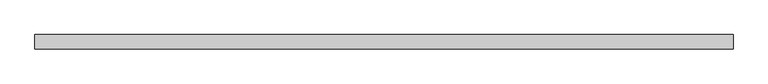
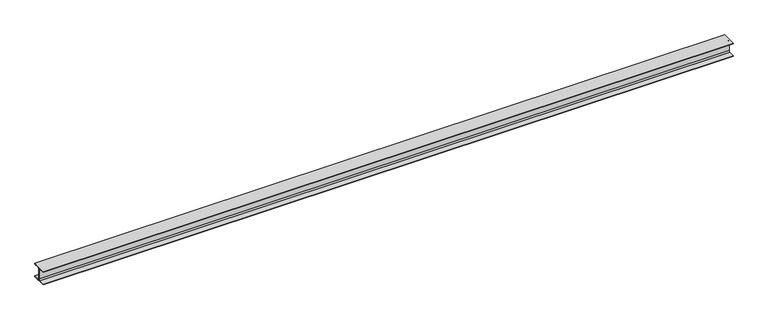
"""IFC4 building model written with IfcOpenShell, lengths in millimetres: beam geometry, NLRS_28_SF_LIB_stalen ligger HEB-AV-CWV-MMBS-SRP_gen_rsf : stalen ligger_gen__HEB 260."""

import ifcopenshell
import ifcopenshell.guid

model = None  # the IFC model being written
_history = None  # IfcOwnerHistory: only IFC2X3 demands one
_inside = {}  # id of a spatial element -> (the spatial element, [elements in it])
_under = {}  # id of a project, library or spatial element -> (it, [spatial elements below it])
_declared = {}  # id of a project -> (the project, [libraries it declares])
_typed = {}  # id of a type object -> (the type object, [elements of that type])
_made_of = {}  # id of a material, layer set ... -> (it, [elements and type objects made of it])


def new_model(schema):
    """Start an empty IFC model of exactly this schema.

    Asked for "IFC4X3", IfcOpenShell would pick the latest addendum, in which some entities
    have other attributes; the version numbers below select the first issue.
    IFC2X3 requires an IfcOwnerHistory on every rooted entity: one is made here for all.
    """
    global model, _history
    if schema == "IFC4X3":
        model = ifcopenshell.file(schema_version=(4, 3, 0, 0))
    else:
        model = ifcopenshell.file(schema=schema)
    _inside.clear()
    _under.clear()
    _declared.clear()
    _typed.clear()
    _made_of.clear()
    _history = None
    if model.schema == "IFC2X3":
        org = make("IfcOrganization", Name="unknown")
        user = make(
            "IfcPersonAndOrganization",
            ThePerson=make("IfcPerson", FamilyName="unknown"),
            TheOrganization=org,
        )
        app = make(
            "IfcApplication",
            ApplicationDeveloper=org,
            Version="unknown",
            ApplicationFullName="unknown",
            ApplicationIdentifier="unknown",
        )
        _history = make(
            "IfcOwnerHistory",
            OwningUser=user,
            OwningApplication=app,
            ChangeAction="ADDED",
            CreationDate=0,
        )
    return model


def make(cls, **values):
    """One entity of the class cls with the attributes given. An attribute that is None is left unset."""
    return model.create_entity(
        cls, **{name: value for name, value in values.items() if value is not None}
    )


def rooted(cls, **values):
    """An entity with a GlobalId (a new one), such as an element, a storey or a relation."""
    return make(cls, GlobalId=ifcopenshell.guid.new(), OwnerHistory=_history, **values)


def si_unit(unit_type, name, prefix=None):
    """IfcSIUnit, for example si_unit("LENGTHUNIT", "METRE", prefix="MILLI")."""
    return make("IfcSIUnit", UnitType=unit_type, Prefix=prefix, Name=name)


def assignment(units):
    """IfcUnitAssignment: the units of a project."""
    return None if units is None else make("IfcUnitAssignment", Units=units)


def point(xyz):
    """IfcCartesianPoint."""
    return None if xyz is None else make("IfcCartesianPoint", Coordinates=xyz)


def direction(xyz):
    """IfcDirection."""
    return None if xyz is None else make("IfcDirection", DirectionRatios=xyz)


def frame(location, z_axis=None, x_axis=None):
    """IfcAxis2Placement3D, a coordinate frame: its origin and axes. An axis left out is left unset."""
    return make(
        "IfcAxis2Placement3D",
        Location=point(location),
        Axis=direction(z_axis),
        RefDirection=direction(x_axis),
    )


def frame_2d(location, x_axis=None):
    """IfcAxis2Placement2D, a coordinate frame in the plane: its origin and x axis."""
    return make(
        "IfcAxis2Placement2D", Location=point(location), RefDirection=direction(x_axis)
    )


def origin():
    """The frame at (0, 0, 0) with its axes left unset."""
    return frame((0.0, 0.0, 0.0))


def place(relative_to, where):
    """IfcLocalPlacement: puts the frame where relative to a parent placement (None: the world)."""
    return make(
        "IfcLocalPlacement", PlacementRelTo=relative_to, RelativePlacement=where
    )


def context(
    kind, dimensions, precision=None, world=None, true_north=None, identifier=None
):
    """IfcGeometricRepresentationContext, for example the 3D "Model" context."""
    return make(
        "IfcGeometricRepresentationContext",
        ContextIdentifier=identifier,
        ContextType=kind,
        CoordinateSpaceDimension=dimensions,
        Precision=precision,
        WorldCoordinateSystem=world,
        TrueNorth=true_north,
    )


def project(units=None, contexts=None):
    """IfcProject with its units and contexts."""
    return rooted(
        "IfcProject",
        Name="project",
        RepresentationContexts=contexts,
        UnitsInContext=assignment(units),
    )


def spatial(cls, under=None, at=None, **own):
    """A site, building, storey or space (cls), placed at a placement, below another one or the project."""
    s = rooted(cls, ObjectPlacement=at, **own)
    if under is not None:
        _under.setdefault(under.id(), (under, []))[1].append(s)
    return s


def polyline(points):
    """IfcPolyline through the points."""
    return make("IfcPolyline", Points=[point(p) for p in points])


def circle_curve(where, radius):
    """IfcCircle in the frame where."""
    return make("IfcCircle", Position=where, Radius=radius)


def trimmed(basis, trim1, trim2, sense, master):
    """IfcTrimmedCurve: the piece of a basis curve between two trims."""
    return make(
        "IfcTrimmedCurve",
        BasisCurve=basis,
        Trim1=trim1,
        Trim2=trim2,
        SenseAgreement=sense,
        MasterRepresentation=master,
    )


def segment(curve, same_sense, transition):
    """IfcCompositeCurveSegment."""
    return make(
        "IfcCompositeCurveSegment",
        Transition=transition,
        SameSense=same_sense,
        ParentCurve=curve,
    )


def composite_curve(segments, self_intersect=None):
    """IfcCompositeCurve: segments joined end to end."""
    return make("IfcCompositeCurve", Segments=segments, SelfIntersect=self_intersect)


def outline(outer, holes=None, kind="AREA"):
    """IfcArbitraryClosedProfileDef: a profile drawn as a closed curve; with holes, ...WithVoids."""
    if holes is None:
        return make("IfcArbitraryClosedProfileDef", ProfileType=kind, OuterCurve=outer)
    return make(
        "IfcArbitraryProfileDefWithVoids",
        ProfileType=kind,
        OuterCurve=outer,
        InnerCurves=holes,
    )


def extrude(swept, where, along, depth):
    """IfcExtrudedAreaSolid: the profile swept, set in the frame where, extruded along a direction by depth."""
    return make(
        "IfcExtrudedAreaSolid",
        SweptArea=swept,
        Position=where,
        ExtrudedDirection=direction(along),
        Depth=depth,
    )


def shape(context_of_items, identifier, shape_type, items):
    """IfcShapeRepresentation: the items that make up one representation, for example the "Body"."""
    return make(
        "IfcShapeRepresentation",
        ContextOfItems=context_of_items,
        RepresentationIdentifier=identifier,
        RepresentationType=shape_type,
        Items=items,
    )


def source(mapping_origin, context_of_items, identifier, shape_type, items):
    """IfcRepresentationMap: a shape defined once, which mapped items show again and again."""
    return make(
        "IfcRepresentationMap",
        MappingOrigin=mapping_origin,
        MappedRepresentation=shape(context_of_items, identifier, shape_type, items),
    )


def transform(
    local_origin,
    x_axis=None,
    y_axis=None,
    z_axis=None,
    scale=None,
    scale2=None,
    scale3=None,
    uniform=True,
):
    """IfcCartesianTransformationOperator3D, or its non-uniform kind. x_axis, y_axis, z_axis: its Axis1, 2, 3."""
    if uniform:
        return make(
            "IfcCartesianTransformationOperator3D",
            Axis1=direction(x_axis),
            Axis2=direction(y_axis),
            LocalOrigin=point(local_origin),
            Scale=scale,
            Axis3=direction(z_axis),
        )
    return make(
        "IfcCartesianTransformationOperator3DnonUniform",
        Axis1=direction(x_axis),
        Axis2=direction(y_axis),
        LocalOrigin=point(local_origin),
        Scale=scale,
        Axis3=direction(z_axis),
        Scale2=scale2,
        Scale3=scale3,
    )


def mapped(mapping_source, mapping_target):
    """IfcMappedItem: shows the shape of a source again, moved by a transform."""
    return make(
        "IfcMappedItem", MappingSource=mapping_source, MappingTarget=mapping_target
    )


def made_of(thing, what):
    """Note that an element or type object is made of a material, layer set ...; save() writes the relation."""
    if what is not None:
        _made_of.setdefault(what.id(), (what, []))[1].append(thing)
    return thing


def element(
    cls,
    number,
    at=None,
    inside=None,
    cuts=None,
    type_object=None,
    material=None,
    context=None,
    identifier="Body",
    shape_type=None,
    held_by="IfcProductDefinitionShape",
    body=None,
    shapes=None,
    **own,
):
    """One element of the class cls, such as IfcWall. Its Tag is "e" and its number.

    at: its placement. inside: the storey or other place that contains it. cuts: it is an
    opening in that element (IfcRelVoidsElement). A single representation is given by context,
    identifier, shape_type and body (its items); several are given by shapes. held_by: the class
    of the entity that holds the representations. save() writes the other relations.
    """
    e = rooted(cls, Tag="e%d" % number, ObjectPlacement=at, **own)
    if body is not None:
        shapes = [shape(context, identifier, shape_type, body)]
    if shapes is not None:
        e.Representation = make(held_by, Representations=shapes)
    if inside is not None:
        _inside.setdefault(inside.id(), (inside, []))[1].append(e)
    if cuts is not None:
        rooted(
            "IfcRelVoidsElement", RelatingBuildingElement=cuts, RelatedOpeningElement=e
        )
    if type_object is not None:
        _typed.setdefault(type_object.id(), (type_object, []))[1].append(e)
    return made_of(e, material)


def aggregate(whole, parts):
    """IfcRelAggregates: a whole, such as a stair, and the parts it consists of."""
    return rooted("IfcRelAggregates", RelatingObject=whole, RelatedObjects=parts)


def save(model, path):
    """Write the relations noted so far, then the file.

    IfcRelAggregates (storeys below a building ...), IfcRelContainedInSpatialStructure (elements
    in a storey), IfcRelDefinesByType, IfcRelAssociatesMaterial and IfcRelDeclares: one each for
    every whole, place, type object, material and project.
    """
    for whole, parts in _under.values():
        aggregate(whole, parts)
    for where, things in _inside.values():
        rooted(
            "IfcRelContainedInSpatialStructure",
            RelatedElements=things,
            RelatingStructure=where,
        )
    for kind, things in _typed.values():
        rooted("IfcRelDefinesByType", RelatedObjects=things, RelatingType=kind)
    for what, things in _made_of.values():
        rooted("IfcRelAssociatesMaterial", RelatedObjects=things, RelatingMaterial=what)
    for by, libraries in _declared.values():
        rooted("IfcRelDeclares", RelatingContext=by, RelatedDefinitions=libraries)
    model.write(path)


def beam_0ced8335(model_context):
    return source(origin(), model_context, "Body", "SweptSolid", [
        extrude(outline(composite_curve([segment(polyline([(130.0, 112.5), (29.0, 112.5)]), True, "CONTINUOUS"), segment(trimmed(circle_curve(frame_2d((29.0, 88.5)), 24.0), [point((29.0, 112.5))], [point((5.0, 88.5))], True, "CARTESIAN"), True, "CONTINUOUS"), segment(polyline([(5.0, 88.5), (5.0, -88.5)]), True, "CONTINUOUS"), segment(trimmed(circle_curve(frame_2d((29.0, -88.5)), 24.0), [point((5.0, -88.5))], [point((29.0, -112.5))], True, "CARTESIAN"), True, "CONTINUOUS"), segment(polyline([(29.0, -112.5), (130.0, -112.5), (130.0, -130.0), (-130.0, -130.0), (-130.0, -112.5), (-29.0, -112.5)]), True, "CONTINUOUS"), segment(trimmed(circle_curve(frame_2d((-29.0, -88.5)), 24.0), [point((-29.0, -112.5))], [point((-5.0, -88.5))], True, "CARTESIAN"), True, "CONTINUOUS"), segment(polyline([(-5.0, -88.5), (-5.0, 88.5)]), True, "CONTINUOUS"), segment(trimmed(circle_curve(frame_2d((-29.0, 88.5)), 24.0), [point((-5.0, 88.5))], [point((-29.0, 112.5))], True, "CARTESIAN"), True, "CONTINUOUS"), segment(polyline([(-29.0, 112.5), (-130.0, 112.5), (-130.0, 130.0), (130.0, 130.0), (130.0, 112.5)]), True, "CONTINUOUS")], self_intersect=False)), frame((-6318.75, 0.0, 0.0), z_axis=(1.0, 0.0, 0.0), x_axis=(0.0, 1.0, 0.0)), (0.0, 0.0, 1.0), 12637.5),
    ])


if __name__ == "__main__":
    model = new_model("IFC4")
    model_context = context("Model", 3, world=origin())
    ifc_project = project(units=[si_unit("LENGTHUNIT", "METRE", prefix="MILLI")], contexts=[model_context])
    site = spatial("IfcSite", under=ifc_project)
    building = spatial("IfcBuilding", under=site)
    placement = place(None, origin())
    beam_shape = beam_0ced8335(model_context)
    element("IfcBeam", 1, ObjectType="NLRS_28_SF_LIB_stalen ligger HEB-AV-CWV-MMBS-SRP_gen_rsf : stalen ligger_gen__HEB 260", at=placement, inside=building, context=model_context, shape_type="MappedRepresentation", body=[
        mapped(beam_shape, transform((0.0, 0.0, 0.0), x_axis=(1.0, 0.0, 0.0), y_axis=(0.0, 1.0, 0.0), z_axis=(0.0, 0.0, 1.0))),
    ])
    save(model, "model.ifc")

# Revit data of these elements
# Type "NLRS_28_SF_LIB_stalen ligger HEB-AV-CWV-MMBS-SRP_gen_rsf : stalen ligger_gen__HEB 260"
#   Type IfcGUID = "0zo1UjqZ91lRsfCKsOOa5a"
#   IfcExportAs = "IfcBeamType"
#   Type Comments = "HEB260"
#   Model = " "
#   Manufacturer = " "
#   Fire Rating = " "
#   Description = "stalen ligger HEB260"
#   Assembly Code = "28.11"
#   ra = 24 mm
#   vz = 130 mm
#   vy = 130 mm
#   vpz = 130 mm
#   vpy = 130 mm
#   NLRS_C_lengte [instance default] = 1500 mm
#   Length [instance default] = 1500 mm
#   bf = 260 mm
#   d = 260 mm
#   tf = 17.5 mm
#   tw = 10 mm
#   Structural Material = NLRS_h2_staal_gen_rsf
#   Keynote = ""
# Element 1 (IfcBeam, "NLRS_28_SF_LIB_stalen ligger HEB-AV-CWV-MMBS-SRP_gen_rsf : stalen ligger_gen__HEB 260")
#   NLRS_C_lengte = 12637.5 mm
#   Materials on its faces: "NLRS_h2_staal_gen_rsf"
# Materials
#   "NLRS_h2_staal_gen_rsf": class "H - Metaal", colour RGB 189 187 185, transparency 0, Keynote = "h2", Manufacturer = "Revit Standards Foundation", URL = "www.revitstandards.org", Description = "staal", Cost = 0
